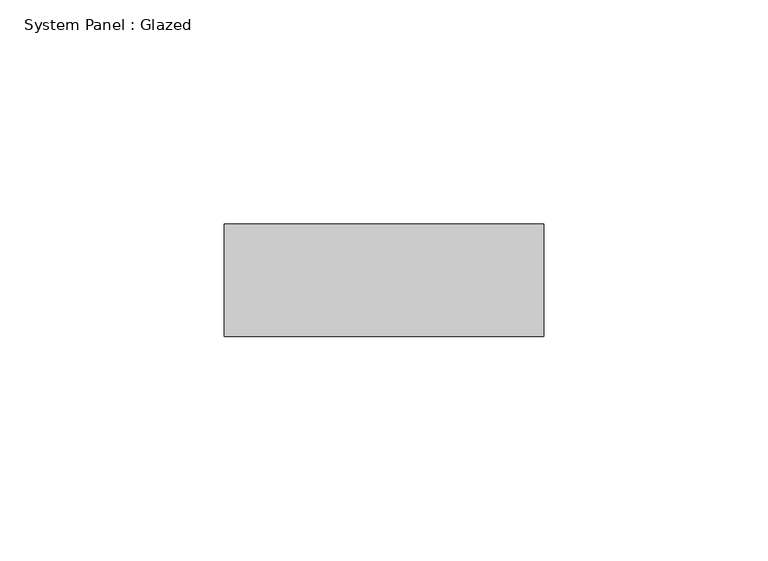
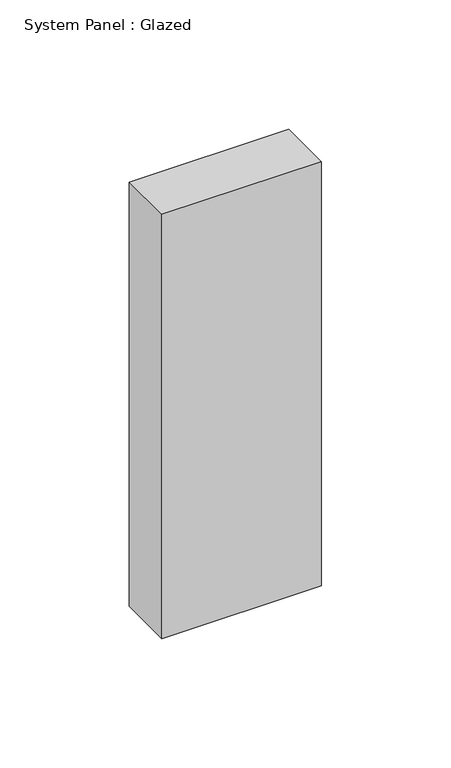
"""IFC4 building model written with IfcOpenShell, lengths in millimetres: plate geometry, System Panel : Glazed."""

from ifc_helpers import new_model, si_unit, origin, origin_with_axes, place, context, project, spatial, polyline, outline, extrude, source, transform, mapped, element, save


def system_panel_glazed_d81ce811(model_context):
    return source(origin(), model_context, "Body", "SweptSolid", [
        extrude(outline(polyline([(35.5642182, 24.5), (-35.5642182, 24.5), (-35.5642182, 49.5), (35.5642182, 49.5), (35.5642182, 24.5)])), origin_with_axes(), (0.0, 0.0, 1.0), 200.0),
    ])


if __name__ == "__main__":
    model = new_model("IFC4")
    model_context = context("Model", 3, world=origin())
    ifc_project = project(units=[si_unit("LENGTHUNIT", "METRE", prefix="MILLI")], contexts=[model_context])
    site = spatial("IfcSite", under=ifc_project)
    building = spatial("IfcBuilding", under=site)
    placement = place(None, origin())
    system_panel_glazed_shape = system_panel_glazed_d81ce811(model_context)
    element("IfcPlate", 1, ObjectType="System Panel : Glazed", at=placement, inside=building, context=model_context, shape_type="MappedRepresentation", body=[
        mapped(system_panel_glazed_shape, transform((0.0, 0.0, 0.0), x_axis=(1.0, 0.0, 0.0), y_axis=(0.0, 1.0, 0.0), z_axis=(0.0, 0.0, 1.0))),
    ])
    save(model, "model.ifc")

# Revit data of these elements
# Element 1 (IfcPlate, "System Panel : Glazed")
#   Materials on its faces: "Glass"
# Materials
#   "Glass": class "Glass", colour RGB 218 227 224, transparency 0.85, Description = "Soda Lime Glass", Cost = 0
